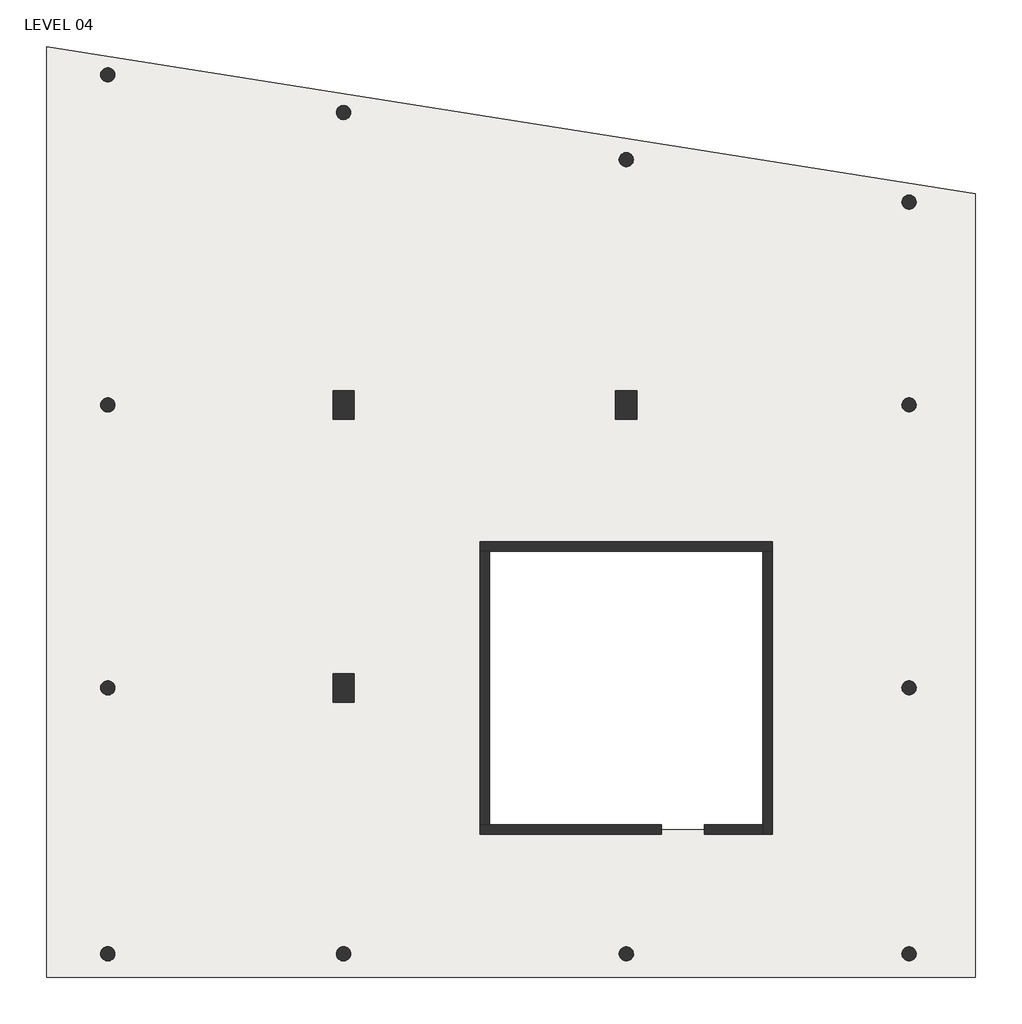
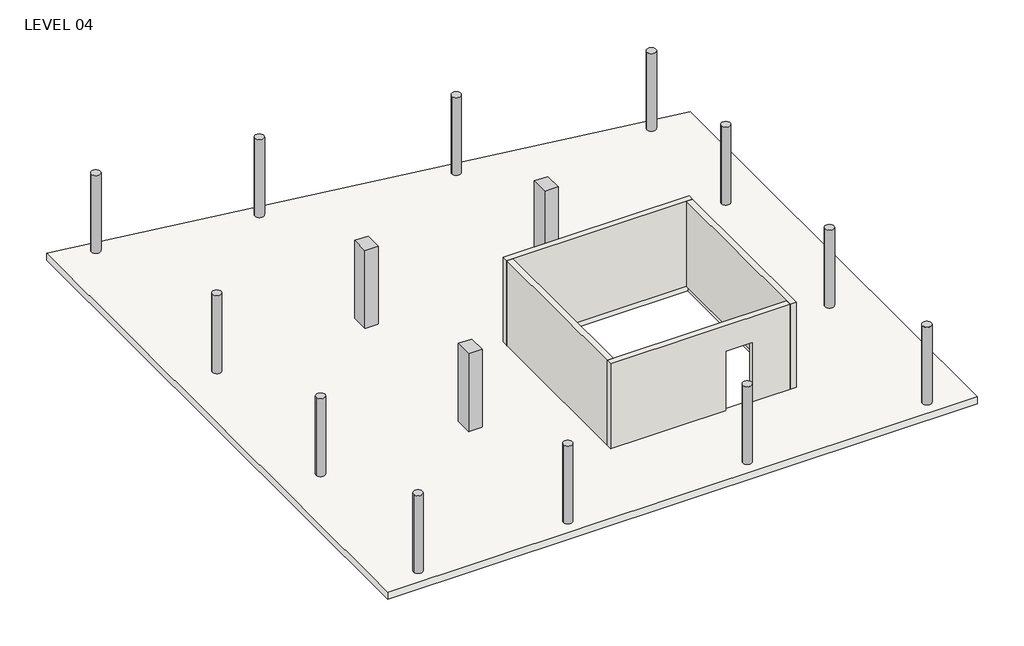
# One storey: 15 columns, 4 beams, 4 walls, 1 slab.
"""IFC4 building model written with IfcOpenShell, lengths in millimetres."""

from ifc_helpers import new_model, si_unit, point, frame, frame_2d, origin, place, context, project, spatial, polyline, circle_curve, trimmed, segment, composite_curve, outline, extrude, faceted_brep, element, save

model = new_model("IFC4")

# Units and contexts
model_context = context("Model", 3, world=origin())
ifc_project = project(units=[si_unit("LENGTHUNIT", "METRE", prefix="MILLI")], contexts=[model_context])

# Site, building, storey
site = spatial("IfcSite", under=ifc_project)
building = spatial("IfcBuilding", under=site)
storey = spatial("IfcBuildingStorey", under=building, Name="LEVEL 04", Elevation=12000.0)

# Beams
placement = place(None, origin())
element("IfcBeam", 1, ObjectType="BHm_StructuralFraming_Concrete-RectangularBeam : 300x500 DP RC BEAM", at=placement, inside=storey, context=model_context, shape_type="SweptSolid", body=[
    extrude(outline(composite_curve([segment(polyline([(-15925.1680269, 21640.7845261), (-15925.1680269, 14640.7845261)]), True, "CONTINUOUS"), segment(trimmed(circle_curve(frame_2d((-16075.1680269, 14640.7845261)), 150.0), [point((-15925.1680269, 14640.7845261))], [point((-16225.1680269, 14640.7845261))], True, "CARTESIAN"), True, "CONTINUOUS"), segment(polyline([(-16225.1680269, 14640.7845261), (-16225.1680269, 21640.7845261)]), True, "CONTINUOUS"), segment(trimmed(circle_curve(frame_2d((-16075.1680269, 21640.7845261)), 150.0), [point((-16225.1680269, 21640.7845261))], [point((-15925.1680269, 21640.7845261))], True, "CARTESIAN"), True, "CONTINUOUS")], self_intersect=False)), frame((0.0, 0.0, 11500.0), z_axis=(0.0, 0.0, 1.0), x_axis=(1.0, 0.0, 0.0)), (0.0, 0.0, 1.0), 250.0),
])
element("IfcBeam", 2, ObjectType="BHm_StructuralFraming_Concrete-RectangularBeam : 300x500 DP RC BEAM", at=placement, inside=storey, context=model_context, shape_type="SweptSolid", body=[
    extrude(outline(composite_curve([segment(polyline([(-10925.1680269, 20840.7845261), (-10925.1680269, 14940.7845261), (-11225.1680269, 14940.7845261), (-11225.1680269, 20840.7845261)]), True, "CONTINUOUS"), segment(trimmed(circle_curve(frame_2d((-11075.1680269, 20840.7845261)), 150.0), [point((-11225.1680269, 20840.7845261))], [point((-10925.1680269, 20840.7845261))], True, "CARTESIAN"), True, "CONTINUOUS")], self_intersect=False)), frame((0.0, 0.0, 11500.0), z_axis=(0.0, 0.0, 1.0), x_axis=(1.0, 0.0, 0.0)), (0.0, 0.0, 1.0), 250.0),
])
element("IfcBeam", 3, ObjectType="BHm_StructuralFraming_Concrete-RectangularBeam : 300x500 DP RC BEAM", at=placement, inside=storey, context=model_context, shape_type="SweptSolid", body=[
    extrude(outline(composite_curve([segment(polyline([(-4925.1680269, 19840.7845261), (-4925.1680269, 14940.7845261), (-5225.1680269, 14940.7845261), (-5225.1680269, 19840.7845261)]), True, "CONTINUOUS"), segment(trimmed(circle_curve(frame_2d((-5075.1680269, 19840.7845261)), 150.0), [point((-5225.1680269, 19840.7845261))], [point((-4925.1680269, 19840.7845261))], True, "CARTESIAN"), True, "CONTINUOUS")], self_intersect=False)), frame((0.0, 0.0, 11500.0), z_axis=(0.0, 0.0, 1.0), x_axis=(1.0, 0.0, 0.0)), (0.0, 0.0, 1.0), 250.0),
])
element("IfcBeam", 4, ObjectType="BHm_StructuralFraming_Concrete-RectangularBeam : 300x500 DP RC BEAM", at=placement, inside=storey, context=model_context, shape_type="SweptSolid", body=[
    extrude(outline(composite_curve([segment(polyline([(1074.8319731, 18940.7845261), (1074.8319731, 14640.7845261)]), True, "CONTINUOUS"), segment(trimmed(circle_curve(frame_2d((924.8319731, 14640.7845261)), 150.0), [point((1074.8319731, 14640.7845261))], [point((774.8319731, 14640.7845261))], True, "CARTESIAN"), True, "CONTINUOUS"), segment(polyline([(774.8319731, 14640.7845261), (774.8319731, 18940.7845261)]), True, "CONTINUOUS"), segment(trimmed(circle_curve(frame_2d((924.8319731, 18940.7845261)), 150.0), [point((774.8319731, 18940.7845261))], [point((1074.8319731, 18940.7845261))], True, "CARTESIAN"), True, "CONTINUOUS")], self_intersect=False)), frame((0.0, 0.0, 11500.0), z_axis=(0.0, 0.0, 1.0), x_axis=(1.0, 0.0, 0.0)), (0.0, 0.0, 1.0), 250.0),
])

# Columns
element("IfcColumn", 5, ObjectType="BHm_StructuralColumns_ConcreteRound : 300 Ø RC COL", at=placement, inside=storey, context=model_context, shape_type="SweptSolid", body=[
    extrude(outline(composite_curve([segment(trimmed(circle_curve(frame_2d((-5075.1680269, 3000.0)), 150.0), [point((-5225.1680269, 3000.0))], [point((-4925.1680269, 3000.0))], False, "CARTESIAN"), True, "CONTINUOUS"), segment(trimmed(circle_curve(frame_2d((-5075.1680269, 3000.0)), 150.0), [point((-4925.1680269, 3000.0))], [point((-5225.1680269, 3000.0))], False, "CARTESIAN"), True, "CONTINUOUS")], self_intersect=False)), frame((0.0, 0.0, 12000.0), z_axis=(0.0, 0.0, 1.0), x_axis=(1.0, 0.0, 0.0)), (0.0, 0.0, 1.0), 2750.0),
])
element("IfcColumn", 6, ObjectType="BHm_StructuralColumns_ConcreteRound : 300 Ø RC COL", at=placement, inside=storey, context=model_context, shape_type="SweptSolid", body=[
    extrude(outline(composite_curve([segment(trimmed(circle_curve(frame_2d((924.8319731, 14640.7845261)), 150.0), [point((774.8319731, 14640.7845261))], [point((1074.8319731, 14640.7845261))], False, "CARTESIAN"), True, "CONTINUOUS"), segment(trimmed(circle_curve(frame_2d((924.8319731, 14640.7845261)), 150.0), [point((1074.8319731, 14640.7845261))], [point((774.8319731, 14640.7845261))], False, "CARTESIAN"), True, "CONTINUOUS")], self_intersect=False)), frame((0.0, 0.0, 12000.0), z_axis=(0.0, 0.0, 1.0), x_axis=(1.0, 0.0, 0.0)), (0.0, 0.0, 1.0), 2750.0),
])
element("IfcColumn", 7, ObjectType="BHm_StructuralColumns_ConcreteRound : 300 Ø RC COL", at=placement, inside=storey, context=model_context, shape_type="SweptSolid", body=[
    extrude(outline(composite_curve([segment(trimmed(circle_curve(frame_2d((924.8319731, 8640.7845261)), 150.0), [point((774.8319731, 8640.7845261))], [point((1074.8319731, 8640.7845261))], False, "CARTESIAN"), True, "CONTINUOUS"), segment(trimmed(circle_curve(frame_2d((924.8319731, 8640.7845261)), 150.0), [point((1074.8319731, 8640.7845261))], [point((774.8319731, 8640.7845261))], False, "CARTESIAN"), True, "CONTINUOUS")], self_intersect=False)), frame((0.0, 0.0, 12000.0), z_axis=(0.0, 0.0, 1.0), x_axis=(1.0, 0.0, 0.0)), (0.0, 0.0, 1.0), 2750.0),
])
element("IfcColumn", 8, ObjectType="BHm_StructuralColumns_ConcreteRound : 300 Ø RC COL", at=placement, inside=storey, context=model_context, shape_type="SweptSolid", body=[
    extrude(outline(composite_curve([segment(trimmed(circle_curve(frame_2d((924.8319731, 3000.0)), 150.0), [point((774.8319731, 3000.0))], [point((1074.8319731, 3000.0))], False, "CARTESIAN"), True, "CONTINUOUS"), segment(trimmed(circle_curve(frame_2d((924.8319731, 3000.0)), 150.0), [point((1074.8319731, 3000.0))], [point((774.8319731, 3000.0))], False, "CARTESIAN"), True, "CONTINUOUS")], self_intersect=False)), frame((0.0, 0.0, 12000.0), z_axis=(0.0, 0.0, 1.0), x_axis=(1.0, 0.0, 0.0)), (0.0, 0.0, 1.0), 2750.0),
])
element("IfcColumn", 9, ObjectType="BHm_StructuralColumns_ConcreteRound : 300 Ø RC COL", at=placement, inside=storey, context=model_context, shape_type="SweptSolid", body=[
    extrude(outline(composite_curve([segment(trimmed(circle_curve(frame_2d((-11075.1680269, 3000.0)), 150.0), [point((-11225.1680269, 3000.0))], [point((-10925.1680269, 3000.0))], False, "CARTESIAN"), True, "CONTINUOUS"), segment(trimmed(circle_curve(frame_2d((-11075.1680269, 3000.0)), 150.0), [point((-10925.1680269, 3000.0))], [point((-11225.1680269, 3000.0))], False, "CARTESIAN"), True, "CONTINUOUS")], self_intersect=False)), frame((0.0, 0.0, 12000.0), z_axis=(0.0, 0.0, 1.0), x_axis=(1.0, 0.0, 0.0)), (0.0, 0.0, 1.0), 2750.0),
])
element("IfcColumn", 10, ObjectType="BHm_StructuralColumns_ConcreteRound : 300 Ø RC COL", at=placement, inside=storey, context=model_context, shape_type="SweptSolid", body=[
    extrude(outline(composite_curve([segment(trimmed(circle_curve(frame_2d((-16075.1680269, 14640.7845261)), 150.0), [point((-16225.1680269, 14640.7845261))], [point((-15925.1680269, 14640.7845261))], False, "CARTESIAN"), True, "CONTINUOUS"), segment(trimmed(circle_curve(frame_2d((-16075.1680269, 14640.7845261)), 150.0), [point((-15925.1680269, 14640.7845261))], [point((-16225.1680269, 14640.7845261))], False, "CARTESIAN"), True, "CONTINUOUS")], self_intersect=False)), frame((0.0, 0.0, 12000.0), z_axis=(0.0, 0.0, 1.0), x_axis=(1.0, 0.0, 0.0)), (0.0, 0.0, 1.0), 2750.0),
])
element("IfcColumn", 11, ObjectType="BHm_StructuralColumns_ConcreteRound : 300 Ø RC COL", at=placement, inside=storey, context=model_context, shape_type="SweptSolid", body=[
    extrude(outline(composite_curve([segment(trimmed(circle_curve(frame_2d((-16075.1680269, 8640.7845261)), 150.0), [point((-16225.1680269, 8640.7845261))], [point((-15925.1680269, 8640.7845261))], False, "CARTESIAN"), True, "CONTINUOUS"), segment(trimmed(circle_curve(frame_2d((-16075.1680269, 8640.7845261)), 150.0), [point((-15925.1680269, 8640.7845261))], [point((-16225.1680269, 8640.7845261))], False, "CARTESIAN"), True, "CONTINUOUS")], self_intersect=False)), frame((0.0, 0.0, 12000.0), z_axis=(0.0, 0.0, 1.0), x_axis=(1.0, 0.0, 0.0)), (0.0, 0.0, 1.0), 2750.0),
])
element("IfcColumn", 12, ObjectType="BHm_StructuralColumns_ConcreteRound : 300 Ø RC COL", at=placement, inside=storey, context=model_context, shape_type="SweptSolid", body=[
    extrude(outline(composite_curve([segment(trimmed(circle_curve(frame_2d((-16075.1680269, 3000.0)), 150.0), [point((-16225.1680269, 3000.0))], [point((-15925.1680269, 3000.0))], False, "CARTESIAN"), True, "CONTINUOUS"), segment(trimmed(circle_curve(frame_2d((-16075.1680269, 3000.0)), 150.0), [point((-15925.1680269, 3000.0))], [point((-16225.1680269, 3000.0))], False, "CARTESIAN"), True, "CONTINUOUS")], self_intersect=False)), frame((0.0, 0.0, 12000.0), z_axis=(0.0, 0.0, 1.0), x_axis=(1.0, 0.0, 0.0)), (0.0, 0.0, 1.0), 2750.0),
])
element("IfcColumn", 13, ObjectType="BHm_StructuralColumns_ConcreteRound : 300 Ø RC COL", at=placement, inside=storey, context=model_context, shape_type="SweptSolid", body=[
    extrude(outline(composite_curve([segment(trimmed(circle_curve(frame_2d((-11075.1680269, 20840.7845261)), 150.0), [point((-11225.1680269, 20840.7845261))], [point((-10925.1680269, 20840.7845261))], False, "CARTESIAN"), True, "CONTINUOUS"), segment(trimmed(circle_curve(frame_2d((-11075.1680269, 20840.7845261)), 150.0), [point((-10925.1680269, 20840.7845261))], [point((-11225.1680269, 20840.7845261))], False, "CARTESIAN"), True, "CONTINUOUS")], self_intersect=False)), frame((0.0, 0.0, 12000.0), z_axis=(0.0, 0.0, 1.0), x_axis=(1.0, 0.0, 0.0)), (0.0, 0.0, 1.0), 2750.0),
])
element("IfcColumn", 14, ObjectType="BHm_StructuralColumns_ConcreteRound : 300 Ø RC COL", at=placement, inside=storey, context=model_context, shape_type="SweptSolid", body=[
    extrude(outline(composite_curve([segment(trimmed(circle_curve(frame_2d((-5075.1680269, 19840.7845261)), 150.0), [point((-5225.1680269, 19840.7845261))], [point((-4925.1680269, 19840.7845261))], False, "CARTESIAN"), True, "CONTINUOUS"), segment(trimmed(circle_curve(frame_2d((-5075.1680269, 19840.7845261)), 150.0), [point((-4925.1680269, 19840.7845261))], [point((-5225.1680269, 19840.7845261))], False, "CARTESIAN"), True, "CONTINUOUS")], self_intersect=False)), frame((0.0, 0.0, 12000.0), z_axis=(0.0, 0.0, 1.0), x_axis=(1.0, 0.0, 0.0)), (0.0, 0.0, 1.0), 2750.0),
])
element("IfcColumn", 15, ObjectType="BHm_StructuralColumns_ConcreteRound : 300 Ø RC COL", at=placement, inside=storey, context=model_context, shape_type="SweptSolid", body=[
    extrude(outline(composite_curve([segment(trimmed(circle_curve(frame_2d((924.8319731, 18940.7845261)), 150.0), [point((774.8319731, 18940.7845261))], [point((1074.8319731, 18940.7845261))], False, "CARTESIAN"), True, "CONTINUOUS"), segment(trimmed(circle_curve(frame_2d((924.8319731, 18940.7845261)), 150.0), [point((1074.8319731, 18940.7845261))], [point((774.8319731, 18940.7845261))], False, "CARTESIAN"), True, "CONTINUOUS")], self_intersect=False)), frame((0.0, 0.0, 12000.0), z_axis=(0.0, 0.0, 1.0), x_axis=(1.0, 0.0, 0.0)), (0.0, 0.0, 1.0), 2750.0),
])
element("IfcColumn", 16, ObjectType="BHm_StructuralColumns_ConcreteRound : 300 Ø RC COL", at=placement, inside=storey, context=model_context, shape_type="SweptSolid", body=[
    extrude(outline(composite_curve([segment(trimmed(circle_curve(frame_2d((-16075.1680269, 21640.7845261)), 150.0), [point((-16225.1680269, 21640.7845261))], [point((-15925.1680269, 21640.7845261))], False, "CARTESIAN"), True, "CONTINUOUS"), segment(trimmed(circle_curve(frame_2d((-16075.1680269, 21640.7845261)), 150.0), [point((-15925.1680269, 21640.7845261))], [point((-16225.1680269, 21640.7845261))], False, "CARTESIAN"), True, "CONTINUOUS")], self_intersect=False)), frame((0.0, 0.0, 12000.0), z_axis=(0.0, 0.0, 1.0), x_axis=(1.0, 0.0, 0.0)), (0.0, 0.0, 1.0), 2750.0),
])
element("IfcColumn", 17, ObjectType="BHm_StructuralColumns_ConcreteRectangular : 450x600 RC COL", at=placement, inside=storey, context=model_context, shape_type="SweptSolid", body=[
    extrude(outline(polyline([(-10850.1680269, 14940.7845261), (-10850.1680269, 14340.7845261), (-11300.1680269, 14340.7845261), (-11300.1680269, 14940.7845261), (-10850.1680269, 14940.7845261)])), frame((0.0, 0.0, 12000.0), z_axis=(0.0, 0.0, 1.0), x_axis=(1.0, 0.0, 0.0)), (0.0, 0.0, 1.0), 2750.0),
])
element("IfcColumn", 18, ObjectType="BHm_StructuralColumns_ConcreteRectangular : 450x600 RC COL", at=placement, inside=storey, context=model_context, shape_type="SweptSolid", body=[
    extrude(outline(polyline([(-10850.1680269, 8940.7845261), (-10850.1680269, 8340.7845261), (-11300.1680269, 8340.7845261), (-11300.1680269, 8940.7845261), (-10850.1680269, 8940.7845261)])), frame((0.0, 0.0, 12000.0), z_axis=(0.0, 0.0, 1.0), x_axis=(1.0, 0.0, 0.0)), (0.0, 0.0, 1.0), 2750.0),
])
element("IfcColumn", 19, ObjectType="BHm_StructuralColumns_ConcreteRectangular : 450x600 RC COL", at=placement, inside=storey, context=model_context, shape_type="SweptSolid", body=[
    extrude(outline(polyline([(-4850.1680269, 14940.7845261), (-4850.1680269, 14340.7845261), (-5300.1680269, 14340.7845261), (-5300.1680269, 14940.7845261), (-4850.1680269, 14940.7845261)])), frame((0.0, 0.0, 12000.0), z_axis=(0.0, 0.0, 1.0), x_axis=(1.0, 0.0, 0.0)), (0.0, 0.0, 1.0), 2750.0),
])

# Slab
element("IfcSlab", 20, ObjectType="250 THK RC SLAB", at=placement, inside=storey, context=model_context, shape_type="SweptSolid", body=[
    extrude(outline(polyline([(2324.8319731, 19120.6110517), (2324.8319731, 2500.0), (-17375.1680269, 2500.0), (-17375.1680269, 22240.7845261), (2324.8319731, 19120.6110517)]), holes=[polyline([(-2075.1680269, 11640.7845261), (-8075.1680269, 11640.7845261), (-8075.1680269, 5640.7845261), (-2075.1680269, 5640.7845261), (-2075.1680269, 11640.7845261)])]), frame((0.0, 0.0, 11750.0), z_axis=(0.0, 0.0, 1.0), x_axis=(1.0, 0.0, 0.0)), (0.0, 0.0, 1.0), 250.0),
])

# Walls
element("IfcWall", 21, ObjectType="200 THK R.C. WALL", at=placement, inside=storey, context=model_context, shape_type="Brep", body=[
    faceted_brep([(-8175.1680269, 11540.7845261, 12000.0), (-7975.1680269, 11540.7845261, 12000.0), (-2175.1680269, 11540.7845261, 12000.0), (-1975.1680269, 11540.7845261, 12000.0), (-1975.1680269, 11540.7845261, 15000.0), (-2175.1680269, 11540.7845261, 15000.0), (-7975.1680269, 11540.7845261, 15000.0), (-8175.1680269, 11540.7845261, 15000.0), (-8175.1680269, 11740.7845261, 12000.0), (-8175.1680269, 11740.7845261, 15000.0), (-1975.1680269, 11740.7845261, 15000.0), (-1975.1680269, 11740.7845261, 12000.0)], [[[0, 1, 2, 3, 4, 5, 6, 7]], [[8, 9, 10, 11]], [[3, 2, 1, 0, 8, 11]], [[7, 6, 5, 4, 10, 9]], [[4, 3, 11, 10]], [[0, 7, 9, 8]]]),
])
element("IfcWall", 22, ObjectType="200 THK R.C. WALL", at=placement, inside=storey, context=model_context, shape_type="Brep", body=[
    faceted_brep([(-2175.1680269, 11540.7845261, 12000.0), (-2175.1680269, 5740.7845261, 12000.0), (-2175.1680269, 5540.7845261, 12000.0), (-2175.1680269, 5540.7845261, 15000.0), (-2175.1680269, 5740.7845261, 15000.0), (-2175.1680269, 11540.7845261, 15000.0), (-1975.1680269, 11540.7845261, 12000.0), (-1975.1680269, 11540.7845261, 15000.0), (-1975.1680269, 5540.7845261, 15000.0), (-1975.1680269, 5540.7845261, 12000.0)], [[[0, 1, 2, 3, 4, 5]], [[6, 7, 8, 9]], [[2, 1, 0, 6, 9]], [[5, 4, 3, 8, 7]], [[0, 5, 7, 6]], [[3, 2, 9, 8]]]),
])
element("IfcWall", 23, ObjectType="200 THK R.C. WALL", at=placement, inside=storey, context=model_context, shape_type="Brep", body=[
    faceted_brep([(-2175.1680269, 5740.7845261, 12000.0), (-3417.6680269, 5740.7845261, 12000.0), (-3417.6680269, 5740.7845261, 14100.0), (-4332.6680269, 5740.7845261, 14100.0), (-4332.6680269, 5740.7845261, 12000.0), (-7975.1680269, 5740.7845261, 12000.0), (-8175.1680269, 5740.7845261, 12000.0), (-8175.1680269, 5740.7845261, 15000.0), (-7975.1680269, 5740.7845261, 15000.0), (-2175.1680269, 5740.7845261, 15000.0), (-3417.6680269, 5540.7845261, 14100.0), (-3417.6680269, 5540.7845261, 12000.0), (-2175.1680269, 5540.7845261, 12000.0), (-2175.1680269, 5540.7845261, 15000.0), (-8175.1680269, 5540.7845261, 15000.0), (-8175.1680269, 5540.7845261, 12000.0), (-4332.6680269, 5540.7845261, 12000.0), (-4332.6680269, 5540.7845261, 14100.0)], [[[0, 1, 2, 3, 4, 5, 6, 7, 8, 9]], [[10, 11, 12, 13, 14, 15, 16, 17]], [[16, 15, 6, 5, 4]], [[12, 11, 1, 0]], [[9, 8, 7, 14, 13]], [[0, 9, 13, 12]], [[7, 6, 15, 14]], [[4, 3, 17, 16]], [[2, 1, 11, 10]], [[3, 2, 10, 17]]]),
])
element("IfcWall", 24, ObjectType="200 THK R.C. WALL", at=placement, inside=storey, context=model_context, shape_type="SweptSolid", body=[
    extrude(outline(polyline([(-7975.1680269, 11540.7845261), (-7975.1680269, 5740.7845261), (-8175.1680269, 5740.7845261), (-8175.1680269, 11540.7845261), (-7975.1680269, 11540.7845261)])), frame((0.0, 0.0, 12000.0), z_axis=(0.0, 0.0, 1.0), x_axis=(1.0, 0.0, 0.0)), (0.0, 0.0, 1.0), 3000.0),
])

save(model, "model.ifc")

# Revit data of these elements
# Type "BHm_StructuralFraming_Concrete-RectangularBeam : 300x500 DP RC BEAM"
#   Keynote = "E"
#   BHE_Width = 300.000 mm
#   BHE_Length [instance default] = 1524.000 mm
#   BHE_Height = 500.000 mm
#   Length [instance default] = 1524.000 mm
#   b = 300.000 mm
#   h = 500.000 mm
#   Structural Material [instance default] = none
#   Assembly Code = ""
# Type "BHm_StructuralColumns_ConcreteRound : 300 Ø RC COL"
#   Keynote = "E"
#   b = 300.000 mm
#   BHE_Length [instance default] = 2500.000 mm
#   BHE_Diameter = 300.000 mm
#   Structural Material [instance default] = none
# Type "BHm_StructuralColumns_ConcreteRectangular : 450x600 RC COL"
#   Keynote = "E"
#   b = 450.000 mm
#   h = 600.000 mm
#   BHE_Width = 450.000 mm
#   BHE_Length [instance default] = 2500.000 mm
#   BHE_Height = 600.000 mm
#   Structural Material [instance default] = none
# Type "250 THK RC SLAB"
#   Function = 0
#   Layers, outside or top first: 250.000 mm "BHE_Concrete - Cast In-Place" (function 1)
# Type "200 THK R.C. WALL"
#   Layers, outside or top first: 200.000 mm "BHE_Concrete - Cast In-Place" (function 1)
# Element 1 (IfcBeam, "BHm_StructuralFraming_Concrete-RectangularBeam : 300x500 DP RC BEAM")
#   Comments = ""
#   BHE_Length = 7000.000 mm
#   Structural Material = none
#   Phase Created = New Construction
#   Materials on its faces: "BHE_Concrete - Cast In-Place"
# Element 2 (IfcBeam, "BHm_StructuralFraming_Concrete-RectangularBeam : 300x500 DP RC BEAM")
#   Comments = ""
#   BHE_Length = 6200.000 mm
#   Structural Material = none
#   Phase Created = New Construction
#   Materials on its faces: "BHE_Concrete - Cast In-Place"
# Element 3 (IfcBeam, "BHm_StructuralFraming_Concrete-RectangularBeam : 300x500 DP RC BEAM")
#   Comments = ""
#   BHE_Length = 5200.000 mm
#   Structural Material = none
#   Phase Created = New Construction
#   Materials on its faces: "BHE_Concrete - Cast In-Place"
# Element 4 (IfcBeam, "BHm_StructuralFraming_Concrete-RectangularBeam : 300x500 DP RC BEAM")
#   Comments = ""
#   BHE_Length = 4300.000 mm
#   Structural Material = none
#   Phase Created = New Construction
#   Materials on its faces: "BHE_Concrete - Cast In-Place"
# Elements 5, 6, 7, 8, 9, 10, 11, 12, 13, 14, 15, 16 (IfcColumn, "BHm_StructuralColumns_ConcreteRound : 300 Ø RC COL")
#   Comments = ""
#   Structural Material = none
#   Phase Created = New Construction
#   Materials on its faces: "BHE_Concrete - Cast In-Place"
# Elements 17, 18, 19 (IfcColumn, "BHm_StructuralColumns_ConcreteRectangular : 450x600 RC COL")
#   Comments = ""
#   Structural Material = none
#   Phase Created = New Construction
#   Materials on its faces: "BHE_Concrete - Cast In-Place"
# Element 20 (IfcSlab, "250 THK RC SLAB")
#   Comments = ""
#   built-in parameter 1001955 = -0.15708 (stored number, unit not read)
#   Height Offset From Level = 0.000 mm
#   built-in parameter 1001954 = 1
#   Phase Created = New Construction
#   Materials on its faces: "BHE_Concrete - Cast In-Place"
# Elements 21, 22, 23, 24 (IfcWall, "200 THK R.C. WALL")
#   Comments = ""
#   Top Offset = 0.000 mm
#   Base Offset = 0.000 mm
#   wall height = 3000.000 mm
#   Phase Created = New Construction
#   Base Constraint = LEVEL 04
#   Top Constraint = LEVEL 05
#   Materials on its faces: "BHE_Concrete - Cast In-Place"
# Materials
#   "BHE_Concrete - Cast In-Place": class "Concrete", colour RGB 192 192 192, transparency 0, Cost = 0
